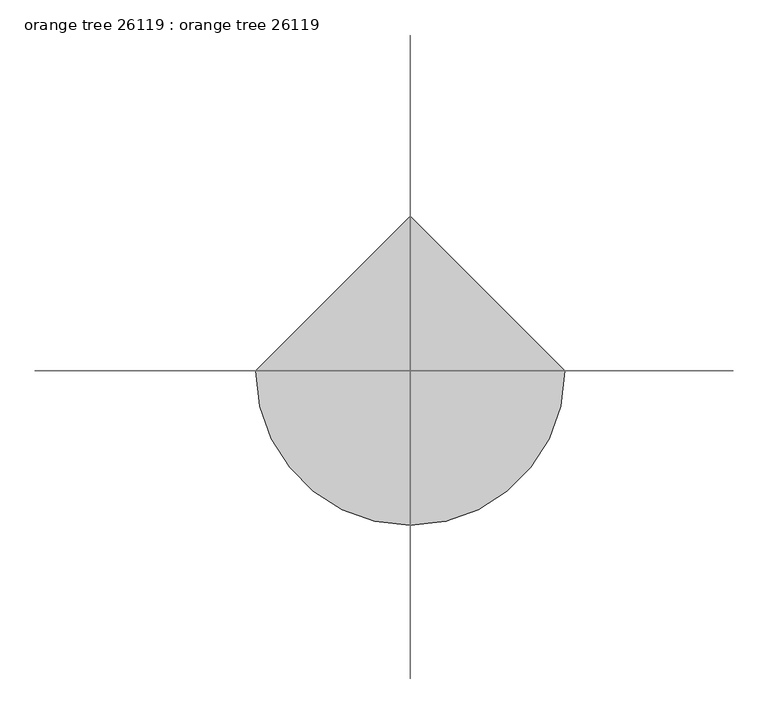
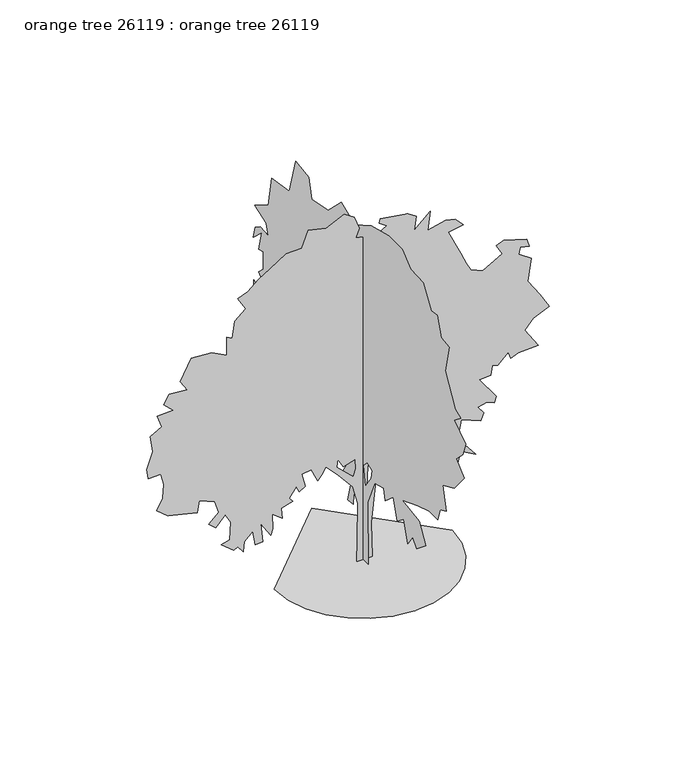
"""IFC4 building model written with IfcOpenShell, lengths in millimetres: proxy geometry, orange tree 26119 : orange tree 26119."""

from ifc_helpers import new_model, si_unit, origin, place, context, project, spatial, triangles, source, transform, mapped, element, save


def orange_tree_26119_orange_tree_26119_d7a228f7(model_context):
    return source(origin(), model_context, "Body", "Tessellation", [
        triangles([(-803.9534712, 0.0, 6.05e-05), (-782.6987366, -184.2127929, 6.05e-05), (-722.1679836, -353.3826814, 6.05e-05), (-627.2075008, -502.663613, 6.05e-05), (-502.663613, -627.2075008, 6.05e-05), (-353.3826814, -722.1679836, 6.05e-05), (-184.2125386, -782.6987366, 6.05e-05), (3.51e-05, -803.9534712, 6.05e-05), (184.2127929, -782.6987366, 6.05e-05), (353.3826814, -722.1679836, 6.05e-05), (502.663613, -627.2075008, 6.05e-05), (627.2075008, -502.663613, 6.05e-05), (722.1679836, -353.3826814, 6.05e-05), (782.6987366, -184.2125386, 6.05e-05), (803.9534712, 7.03e-05, 6.05e-05), (-0.0001054, 803.9534712, 6.05e-05), (-4.73e-05, -77.0963933, 4.81e-05), (-2.95e-05, -72.7562921, 588.9525321), (-2.7e-05, -181.2628458, 836.3460434), (-3.2e-05, -320.1518609, 875.4087753), (-3.63e-05, -346.1919502, 771.2433311), (-3.87e-05, -472.0617019, 879.7495714), (-4.71e-05, -532.8235817, 688.7770712), (-4.92e-05, -632.6507006, 766.9024624), (-5.78e-05, -693.4151602, 571.5916368), (-5.81e-05, -775.878804, 684.4387459), (-6.3e-05, -832.3023949, 606.3134274), (-6.59e-05, -979.8713671, 727.8398031), (-5.62e-05, -875.7059229, 897.110503), (-4.32e-05, -610.9489002, 936.1731623), (-5.12e-05, -849.6633265, 1027.3185436), (-5.75e-05, -1031.9540892, 1088.0830032), (-6.35e-05, -1166.5029985, 1088.0830032), (-6.17e-05, -1201.224789, 1200.9301849), (-6.47e-05, -1296.7111118, 1244.3311695), (-5.59e-05, -1244.6283897, 1461.3462662), (-6.14e-05, -1422.5782837, 1543.8099827), (-6.28e-05, -1578.8289207, 1730.4416142), (-5.38e-05, -1452.9591328, 1843.2887959), (-5.55e-05, -1552.7863243, 1938.7749733), (-5.37e-05, -1600.5281776, 2068.9830139), (-4.21e-05, -1418.2374149, 2186.1685936), (-4.43e-05, -1526.7437279, 2272.9730335), (-3.95e-05, -1439.9391426, 2303.3564987), (-2.42e-05, -1279.3501076, 2576.8055054), (-1.94e-05, -1344.4529652, 2837.2061806), (-1.34e-05, -1218.5857206, 2850.2364899), (-5.3e-06, -1157.821261, 3028.1889999), (-1.5e-06, -1062.3375544, 3015.1586906), (9.7e-06, -940.8087078, 3206.14151), (1.89e-05, -741.1570135, 3214.8028999), (2.81e-05, -606.6080678, 3323.3116837), (3.75e-05, -398.2746723, 3327.6550232), (4.77e-05, -124.839264, 3258.2115875), (5.48e-05, 135.5766083, 3106.2941162), (6.66e-05, 339.5701524, 3197.4545403), (6.98e-05, 543.560172, 2997.8106216), (7.98e-05, 799.6379642, 2950.0585945), (8.73e-05, 847.3798176, 3128.0111046), (9.73e-05, 1051.3723806, 3158.3894829), (9.14e-05, 1151.1994995, 2811.1714325), (0.0001025, 1428.9739689, 2767.7627449), (9.64e-05, 1485.3975597, 2476.9656693), (0.0001018, 1689.3900501, 2351.0983521), (9.21e-05, 1515.7810249, 2285.9956398), (8.75e-05, 1481.0591618, 2186.1685936), (9.36e-05, 1606.926479, 2199.1910545), (9.54e-05, 1685.0517975, 2142.767609), (9.34e-05, 1715.4327919, 2029.9204273), (9.11e-05, 1580.8837372, 2155.7875992), (8.77e-05, 1632.9664593, 1964.815099), (8.51e-05, 1559.1820095, 1986.5168266), (8.02e-05, 1563.5228783, 1817.2460541), (8.14e-05, 1632.9664593, 1752.1433418), (7.34e-05, 1524.4602917, 1647.9754269), (7.38e-05, 1585.2246059, 1569.8525791), (8.13e-05, 1711.0919231, 1630.6144226), (7.79e-05, 1719.7736607, 1504.7472507), (7.16e-05, 1645.9890656, 1404.9226753), (7.48e-05, 1728.4527821, 1387.5618164), (7.27e-05, 1745.813641, 1292.0754936), (6.99e-05, 1650.3299343, 1339.817347), (6.11e-05, 1459.3574341, 1331.1382256), (6.23e-05, 1628.6282066, 1118.463925), (5.81e-05, 1520.1218937, 1140.1657253), (5.99e-05, 1611.2673477, 1062.0404068), (5.99e-05, 1698.0717876, 931.8322935), (5.77e-05, 1637.307328, 949.1932251), (5.11e-05, 1576.5454845, 818.9851845), (5.33e-05, 1572.2046158, 901.4513718), (4.88e-05, 1450.6756966, 931.8322935), (4.52e-05, 1402.9338432, 884.0904402), (4.47e-05, 1281.4075401, 1049.020344), (3.92e-05, 1264.0440651, 888.4313089), (3.71e-05, 1194.6004841, 923.1530994), (3.64e-05, 1116.4751656, 1018.6394222), (2.99e-05, 999.2896585, 975.2358215), (2.55e-05, 955.8861305, 892.7696342), (2.14e-05, 964.567868, 740.8623367), (1.6e-05, 873.4224867, 697.4588087), (1.6e-05, 916.8234713, 632.353553), (1.37e-05, 938.5251989, 523.8472401), (7.6e-06, 743.2143734, 610.6542961), (6.3e-06, 656.4073174, 697.4588087), (2.2e-06, 608.665464, 632.353553), (5.3e-06, 578.2845423, 779.9225252), (9e-07, 521.8609514, 719.1606091), (-7e-07, 456.7556594, 762.5615936), (1.1e-06, 465.4373606, 810.3059904), (-2e-06, 395.9937432, 810.3059904), (-7.3e-06, 335.22932, 723.5014778), (-6e-06, 291.8257738, 832.0077181), (-1e-05, 257.1039651, 749.5415308), (-1.02e-05, 317.8683884, 649.7169554), (-1.72e-05, 122.5560549, 710.4788715), (-1.74e-05, 192.000181, 597.6317262), (-2.03e-05, 244.0831574, 424.0226646), (-2.39e-05, 157.2781179, 432.7018224), (-2.16e-05, 144.2573102, 528.1880725), (-2.27e-05, 92.1740885, 571.5916368), (-2.48e-05, 44.4312178, 571.5916368), (-3.04e-05, 40.0908669, 389.3008378), (-4.11e-05, 61.7923765, 5.22e-05), (-2.23e-05, -137.8603261, 927.4914248), (-2.41e-05, -124.8395184, 849.3686497), (-2.39e-05, -33.6941257, 719.1606091), (-1.71e-05, -3.3121102, 901.4513718), (-1.8e-05, -64.07584, 962.2158314), (58.7260893, 2.69e-05, 920.6994701), (38.9260215, 3.03e-05, 877.8014345), (32.3258294, 4.22e-05, 683.1001648), (45.5259593, 4.5e-05, 626.9992287), (78.5256484, 3.59e-05, 755.7010386), (104.9259083, 2.72e-05, 881.1008698), (-56.7740963, 8.68e-05, 0.0), (-53.4738754, 7.45e-05, 204.6001204), (-50.1739042, 5.35e-05, 554.4008984), (-93.0740155, 4.51e-05, 726.0008165), (-225.0743068, 4.16e-05, 881.1008698), (-337.2739989, 3.93e-05, 1003.2012657), (-363.6747857, 4.36e-05, 950.3996922), (-409.8748363, 4.89e-05, 894.3012995), (-465.9733017, 4.39e-05, 1019.7011307), (-551.7745325, 4.85e-05, 1006.500701), (-522.0743105, 5.46e-05, 881.1008698), (-574.8733043, 5.89e-05, 848.1012125), (-604.5735263, 5.67e-05, 907.4991131), (-667.2734419, 6.47e-05, 818.4009905), (-634.2737846, 6.56e-05, 778.799774), (-739.8743156, 7.2e-05, 749.099552), (-729.9733938, 7.77e-05, 646.8010723), (-819.0740599, 7.74e-05, 716.0998947), (-815.7746246, 8.54e-05, 580.7991417), (-832.2744169, 8.94e-05, 524.7006763), (-924.6745909, 8.52e-05, 663.3008646), (-904.8752907, 9.48e-05, 488.3989677), (-970.8746778, 9.8e-05, 481.8000609), (-997.2754646, 9.11e-05, 617.1008503), (-1069.8737223, 9.86e-05, 544.4999765), (-1079.7746441, 0.0001046, 452.0998389), (-1129.2741663, 0.0001028, 518.0991898), (-1165.5758749, 0.0001058, 495.0004543), (-1281.0748569, 0.0001051, 590.7000635), (-1201.8750401, 0.0001005, 610.4993637), (-1195.2735535, 9.05e-05, 772.2009035), (-1241.4736404, 8.73e-05, 861.2990261), (-1327.2749439, 9.65e-05, 768.9013956), (-1389.9747505, 9.61e-05, 821.7004257), (-1300.8740845, 8.71e-05, 907.4991131), (-1337.1733223, 8.2e-05, 1019.7011307), (-1479.0755619, 8.49e-05, 1075.799596), (-1495.5752815, 9.19e-05, 970.2015358), (-1759.5754463, 9.97e-05, 1032.9014877), (-1858.5744907, 9.91e-05, 1115.4007399), (-1805.7755333, 9.07e-05, 1217.6992195), (-1799.1740467, 8.25e-05, 1349.70061), (-1825.5747608, 7.76e-05, 1451.999017), (-1937.7743076, 8.27e-05, 1448.6996544), (-1950.9746647, 7.78e-05, 1541.0998283), (-1894.8735832, 6.63e-05, 1692.9004463), (-1917.9749348, 5.84e-05, 1841.4015564), (-1815.6739117, 5.04e-05, 1900.7993843), (-1855.2749828, 4.52e-05, 2016.3009098), (-1713.3753593, 3.86e-05, 2022.8997803), (-1799.1740467, 3.75e-05, 2105.4015759), (-1746.3750893, 3.05e-05, 2184.6013927), (-1584.6734768, 2.4e-05, 2174.7003983), (-1650.6754074, 2.1e-05, 2273.6994427), (-1548.3743843, 5.5e-06, 2458.4999359), (-1366.8735443, -1.9e-06, 2448.6014122), (-1228.2732834, -3.6e-06, 2376.0006111), (-1228.2732834, -1.38e-05, 2547.5953697), (-1178.7737612, -1.44e-05, 2521.1995972), (-1158.974461, -2.45e-05, 2676.2973976), (-1056.6733652, -3.39e-05, 2758.7964317), (-1132.5736742, -3.79e-05, 2880.8942116), (-1040.1735003, -4.41e-05, 2917.1908333), (-941.1744558, -5.33e-05, 2999.6901581), (-835.5739248, -6.19e-05, 3065.7047333), (-693.6742287, -7.36e-05, 3158.1101395), (-555.0740041, -7.98e-05, 3161.4119728), (-495.6735237, -9.13e-05, 3309.9005836), (-333.9745637, -9.62e-05, 3273.6039619), (-172.2735144, -0.000108, 3352.8011627), (-79.8736311, -0.0001083, 3290.0884209), (-36.9737765, -0.0001029, 3167.990641), (-66.673751, -9.71e-05, 3092.0952736), (114.8263214, -0.0001024, 3049.1946945), (213.8264105, -0.0001101, 3105.303479), (144.5262982, -0.00011, 3154.8080154), (154.426457, -0.0001128, 3194.4067612), (401.9271747, -0.0001213, 3154.8080154), (477.8274837, -0.0001215, 3102.001355), (461.327655, -0.0001133, 2976.6014511), (606.5267864, -0.0001275, 3108.6053123), (580.126036, -0.0001159, 2933.700872), (745.1270473, -0.0001255, 2973.2996178), (827.6262268, -0.0001279, 2953.5130348), (900.2271006, -0.0001263, 2874.2902542), (768.2257828, -0.000119, 2847.8997139), (877.125749, -0.0001096, 2610.3081116), (929.9273226, -0.0001052, 2498.1010071), (969.525923, -0.0001024, 2422.2006981), (1078.4258892, -0.0001042, 2372.7011032), (1253.3278587, -0.000118, 2474.9995102), (1197.2268499, -0.0001212, 2570.7093658), (1266.525745, -0.000126, 2600.4020302), (1474.4272991, -0.0001312, 2534.4002449), (1497.5260345, -0.0001279, 2461.8017693), (1415.0268551, -0.0001252, 2478.3016342), (1401.826498, -0.0001211, 2418.9011902), (1514.0258995, -0.0001213, 2339.7013733), (1481.0261696, -0.0001075, 2131.7998192), (1593.2257164, -0.0001027, 1970.1008228), (1679.0268745, -9.78e-05, 1824.9016914), (1530.5257645, -8.76e-05, 1762.1992687), (1457.9274342, -7.91e-05, 1673.1010735), (1576.7258514, -7.35e-05, 1491.6002335), (1398.5269901, -6.51e-05, 1481.6993843), (1329.2255516, -6.03e-05, 1451.999017), (1309.4263241, -6.32e-05, 1514.701585), (1213.7267149, -5.39e-05, 1428.9002815), (1160.9276848, -5.24e-05, 1442.1006386), (1151.026763, -4.66e-05, 1352.9999725), (1045.426232, -4.18e-05, 1349.70061), (1197.2268499, -3.59e-05, 1138.4994753), (1180.726985, -3.16e-05, 1079.1015747), (1114.7275978, -3.05e-05, 1108.7992533), (1032.2258749, -2.57e-05, 1088.9999531), (1085.0273758, -2.39e-05, 1019.7011307), (1058.626589, -1.86e-05, 950.3996922), (883.7272356, -1.53e-05, 1023.0005659), (854.0270136, -3.8e-06, 851.4006477), (1012.4265747, 1.3e-06, 650.1005075), (877.125749, 2.7e-06, 726.0008165), (830.9257347, 1.63e-05, 531.2995831), (801.2255127, 1.04e-05, 653.3999428), (745.1270473, 8.7e-06, 722.7013813), (642.8259516, 1.59e-05, 676.5012943), (586.7274862, 2.47e-05, 570.900727), (487.725862, 2.15e-05, 696.3005945), (392.0262528, 1.76e-05, 831.6013475), (349.1256374, 2.48e-05, 742.5006815), (316.1259439, 1.76e-05, 887.6998129), (187.4264049, 2.7e-05, 824.999861), (114.8263214, 3.72e-05, 706.1989729), (71.9262193, 6.15e-05, 329.999443), (81.8261282, 8.08e-05, 0.0001067), (-178.8742198, 3.57e-05, 947.1002569), (-228.3742689, 3.25e-05, 1036.200923), (-238.2741733, 3.73e-05, 963.6001219), (-89.7740443, 3.95e-05, 818.4009905), (-66.6740053, 3.43e-05, 887.6998129), (-73.2739431, 2.91e-05, 980.0999868)], [[15, 16, 1], [14, 15, 1], [14, 1, 2], [13, 14, 2], [13, 2, 3], [13, 3, 4], [12, 13, 4], [11, 12, 4], [11, 4, 5], [11, 5, 6], [11, 6, 7], [11, 7, 8], [11, 8, 9], [11, 9, 10], [126, 17, 18], [88, 89, 90], [68, 69, 70], [67, 68, 70], [83, 84, 85], [86, 87, 88], [126, 18, 19], [125, 126, 19], [113, 114, 115], [104, 105, 106], [63, 64, 65], [80, 81, 82], [79, 80, 82], [66, 67, 70], [24, 25, 26], [101, 102, 103], [110, 111, 112], [42, 43, 44], [70, 71, 72], [20, 21, 22], [100, 101, 103], [116, 117, 118], [116, 118, 119], [76, 77, 78], [22, 23, 24], [93, 94, 95], [93, 95, 96], [76, 78, 79], [91, 92, 93], [45, 46, 47], [116, 119, 120], [115, 116, 120], [26, 27, 28], [26, 28, 29], [26, 29, 30], [24, 26, 30], [22, 24, 30], [123, 17, 126], [122, 123, 126], [121, 122, 126], [73, 74, 75], [79, 82, 83], [76, 79, 83], [37, 38, 39], [124, 125, 19], [59, 60, 61], [58, 59, 61], [106, 107, 108], [106, 108, 109], [66, 70, 72], [124, 19, 20], [34, 35, 36], [47, 48, 49], [100, 103, 104], [115, 120, 121], [115, 121, 126], [115, 126, 127], [40, 41, 42], [39, 40, 42], [32, 33, 34], [113, 115, 127], [112, 113, 127], [61, 62, 63], [55, 56, 57], [98, 99, 100], [98, 100, 104], [98, 104, 106], [86, 88, 90], [86, 90, 91], [85, 86, 91], [85, 91, 93], [83, 85, 93], [75, 76, 83], [36, 37, 39], [49, 50, 51], [83, 93, 96], [32, 34, 36], [97, 98, 106], [31, 32, 36], [42, 44, 45], [97, 106, 109], [51, 52, 53], [75, 83, 96], [75, 96, 97], [61, 63, 65], [61, 65, 66], [58, 61, 66], [57, 58, 66], [75, 97, 109], [73, 75, 109], [72, 73, 109], [66, 72, 109], [57, 66, 109], [57, 109, 110], [57, 110, 112], [57, 112, 127], [57, 127, 128], [55, 57, 128], [54, 55, 128], [53, 54, 128], [51, 53, 128], [49, 51, 128], [47, 49, 128], [45, 47, 128], [42, 45, 128], [39, 42, 128], [36, 39, 128], [31, 36, 128], [30, 31, 128], [30, 128, 124], [30, 124, 20], [30, 20, 22], [135, 130, 131], [130, 135, 136], [130, 136, 137], [135, 131, 132], [253, 254, 255], [255, 256, 257], [130, 137, 138], [272, 129, 130], [272, 130, 138], [129, 272, 273], [262, 263, 264], [214, 215, 216], [272, 138, 139], [271, 272, 139], [271, 139, 140], [159, 160, 161], [150, 151, 152], [153, 154, 155], [152, 153, 155], [162, 163, 164], [218, 219, 220], [237, 238, 239], [228, 229, 230], [227, 228, 230], [191, 192, 193], [141, 142, 143], [148, 149, 150], [259, 260, 261], [182, 183, 184], [217, 218, 220], [161, 162, 164], [270, 271, 140], [129, 273, 274], [195, 196, 197], [268, 135, 132], [267, 268, 132], [266, 267, 132], [266, 132, 133], [265, 266, 133], [265, 133, 134], [246, 247, 248], [245, 246, 248], [234, 235, 236], [140, 141, 143], [225, 226, 227], [225, 227, 230], [225, 230, 231], [167, 168, 169], [166, 167, 169], [239, 240, 241], [145, 146, 147], [144, 145, 147], [255, 257, 258], [253, 255, 258], [171, 172, 173], [237, 239, 241], [216, 217, 220], [245, 248, 249], [250, 251, 252], [249, 250, 252], [155, 156, 157], [155, 157, 158], [210, 211, 212], [209, 210, 212], [177, 178, 179], [243, 244, 245], [201, 202, 203], [184, 185, 186], [184, 186, 187], [274, 269, 270], [173, 174, 175], [171, 173, 175], [159, 161, 164], [177, 179, 180], [158, 159, 164], [158, 164, 165], [155, 158, 165], [171, 175, 176], [180, 181, 182], [188, 189, 190], [187, 188, 190], [187, 190, 191], [231, 232, 233], [245, 249, 252], [212, 213, 214], [209, 212, 214], [203, 204, 205], [203, 205, 206], [203, 206, 207], [201, 203, 207], [264, 265, 134], [208, 209, 214], [241, 242, 243], [225, 231, 233], [224, 225, 233], [233, 234, 236], [224, 233, 236], [224, 236, 237], [224, 237, 241], [224, 241, 243], [223, 224, 243], [223, 243, 245], [152, 155, 165], [152, 165, 166], [259, 261, 262], [258, 259, 262], [253, 258, 262], [252, 253, 262], [252, 262, 264], [245, 252, 264], [223, 245, 264], [223, 264, 134], [223, 134, 129], [223, 129, 274], [223, 274, 270], [222, 223, 270], [221, 222, 270], [220, 221, 270], [216, 220, 270], [214, 216, 270], [208, 214, 270], [207, 208, 270], [201, 207, 270], [200, 201, 270], [199, 200, 270], [198, 199, 270], [197, 198, 270], [195, 197, 270], [194, 195, 270], [193, 194, 270], [191, 193, 270], [191, 270, 140], [191, 140, 143], [191, 143, 144], [187, 191, 144], [184, 187, 144], [182, 184, 144], [180, 182, 144], [177, 180, 144], [176, 177, 144], [171, 176, 144], [170, 171, 144], [170, 144, 147], [169, 170, 147], [166, 169, 147], [152, 166, 147], [152, 147, 148], [152, 148, 150]], closed=False),
    ])


if __name__ == "__main__":
    model = new_model("IFC4")
    model_context = context("Model", 3, world=origin())
    ifc_project = project(units=[si_unit("LENGTHUNIT", "METRE", prefix="MILLI")], contexts=[model_context])
    site = spatial("IfcSite", under=ifc_project)
    building = spatial("IfcBuilding", under=site)
    placement = place(None, origin())
    orange_tree_26119_orange_tree_26119_shape = orange_tree_26119_orange_tree_26119_d7a228f7(model_context)
    element("IfcBuildingElementProxy", 1, Name="orange tree 26119 : orange tree 26119", ObjectType="orange tree 26119 : orange tree 26119", at=placement, inside=building, context=model_context, shape_type="MappedRepresentation", body=[
        mapped(orange_tree_26119_orange_tree_26119_shape, transform((0.0, 0.0, 0.0), x_axis=(1.0, 0.0, 0.0), y_axis=(0.0, 1.0, 0.0), z_axis=(0.0, 0.0, 1.0))),
    ])
    save(model, "model.ifc")

# Revit data of these elements
# Type "orange tree 26119 : orange tree 26119"
#   built-in parameter 1005195 = "RPC-16-FVGW-4XXX-7J75-W000-ST1L-LVER-AU"
#   Height = 0
